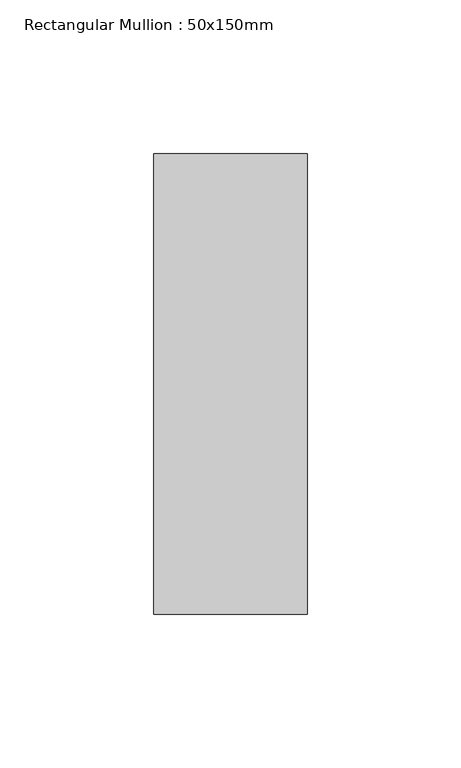
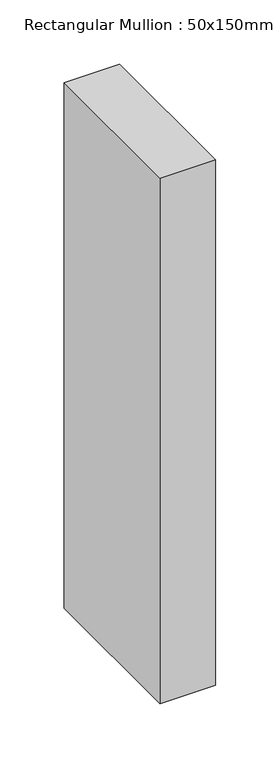
"""IFC4 building model written with IfcOpenShell, lengths in millimetres: member geometry, Rectangular Mullion : 50x150mm."""

from ifc_helpers import new_model, si_unit, frame, origin, place, context, project, spatial, polyline, outline, extrude, source, transform, mapped, element, save


def rectangular_mullion_50x150mm_22f77a7a(model_context):
    return source(origin(), model_context, "Body", "SweptSolid", [
        extrude(outline(polyline([(25.0, 75.0), (25.0, -75.0), (-25.0, -75.0), (-25.0, 75.0), (25.0, 75.0)])), frame((0.0, 0.0, -500.0), z_axis=(0.0, 0.0, 1.0), x_axis=(1.0, 0.0, 0.0)), (0.0, 0.0, 1.0), 500.0),
    ])


if __name__ == "__main__":
    model = new_model("IFC4")
    model_context = context("Model", 3, world=origin())
    ifc_project = project(units=[si_unit("LENGTHUNIT", "METRE", prefix="MILLI")], contexts=[model_context])
    site = spatial("IfcSite", under=ifc_project)
    building = spatial("IfcBuilding", under=site)
    placement = place(None, origin())
    rectangular_mullion_50x150mm_shape = rectangular_mullion_50x150mm_22f77a7a(model_context)
    element("IfcMember", 1, ObjectType="Rectangular Mullion : 50x150mm", at=placement, inside=building, context=model_context, shape_type="MappedRepresentation", body=[
        mapped(rectangular_mullion_50x150mm_shape, transform((0.0, 0.0, 0.0), x_axis=(1.0, 0.0, 0.0), y_axis=(0.0, 1.0, 0.0), z_axis=(0.0, 0.0, 1.0))),
    ])
    save(model, "model.ifc")

# Revit data of these elements
# Type "Rectangular Mullion : 50x150mm"
#   Keynote = "H11"
#   built-in parameter 1007304 = 0.492126 (stored number, unit not read)
#   built-in parameter 1007301 = 0.082021 (stored number, unit not read)
#   built-in parameter 1007300 = 0.082021 (stored number, unit not read)
# Element 1 (IfcMember, "Rectangular Mullion : 50x150mm")
#   Materials on its faces: "Aluminium"
# Materials
#   "Aluminium": class "Metal", colour RGB 247 247 247, transparency 0, Description = "Aluminium 6061", Cost = 0
